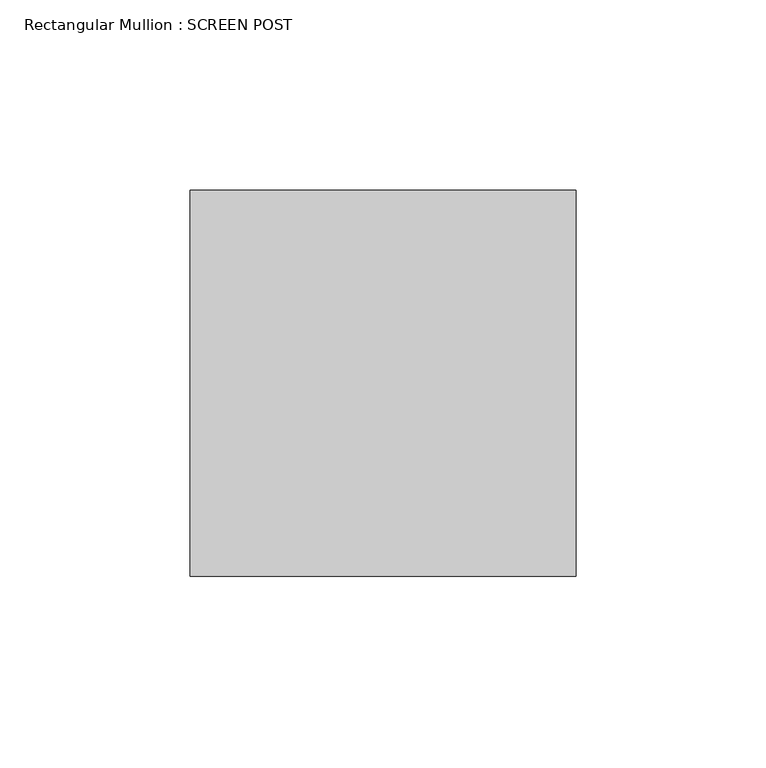
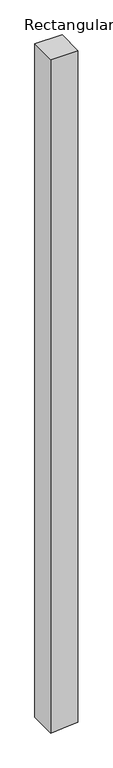
"""IFC4 building model written with IfcOpenShell, lengths in millimetres: member geometry, Rectangular Mullion : SCREEN POST."""

from ifc_helpers import new_model, si_unit, frame, origin, place, context, project, spatial, polyline, outline, extrude, source, transform, mapped, element, save


def rectangular_mullion_screen_post_59f0d0ef(model_context):
    return source(origin(), model_context, "Body", "SweptSolid", [
        extrude(outline(polyline([(0.0, 50.8), (0.0, -50.8), (-2656.4026741, -50.8), (-2653.6194698, -6.3490391), (-2650.0412019, 50.8), (0.0, 50.8)])), frame((0.0, -50.8, 0.0), z_axis=(0.0, 1.0, 0.0), x_axis=(0.0, 0.0, 1.0)), (0.0, 0.0, 1.0), 101.6),
    ])


if __name__ == "__main__":
    model = new_model("IFC4")
    model_context = context("Model", 3, world=origin())
    ifc_project = project(units=[si_unit("LENGTHUNIT", "METRE", prefix="MILLI")], contexts=[model_context])
    site = spatial("IfcSite", under=ifc_project)
    building = spatial("IfcBuilding", under=site)
    placement = place(None, origin())
    rectangular_mullion_screen_post_shape = rectangular_mullion_screen_post_59f0d0ef(model_context)
    element("IfcMember", 1, ObjectType="Rectangular Mullion : SCREEN POST", at=placement, inside=building, context=model_context, shape_type="MappedRepresentation", body=[
        mapped(rectangular_mullion_screen_post_shape, transform((0.0, 0.0, 0.0), x_axis=(1.0, 0.0, 0.0), y_axis=(0.0, 1.0, 0.0), z_axis=(0.0, 0.0, 1.0))),
    ])
    save(model, "model.ifc")

# Revit data of these elements
# Type "Rectangular Mullion : SCREEN POST"
#   built-in parameter 1007304 = 0.333333 (stored number, unit not read)
#   built-in parameter 1007301 = 0.166667 (stored number, unit not read)
#   built-in parameter 1007300 = 0.166667 (stored number, unit not read)
# Element 1 (IfcMember, "Rectangular Mullion : SCREEN POST")
#   Materials on its faces: "GLULAMS COLUMNS\n(PRESSURE TREATED W/ PENTA IN SOLVENT) (EXTERIOR STAIN: PENOFIN VERDE EXT. STAIN - COLOR: CEDAR)"
# Materials
#   "GLULAMS COLUMNS\n(PRESSURE TREATED W/ PENTA IN SOLVENT) (EXTERIOR STAIN: PENOFIN VERDE EXT. STAIN - COLOR: CEDAR)": class "Wood", colour RGB 164 134 123, transparency 0, Description = "Pinus Echinata", Cost = 0
